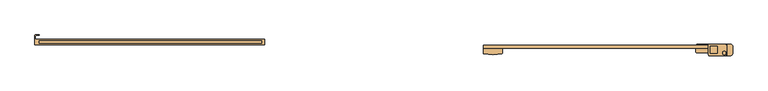
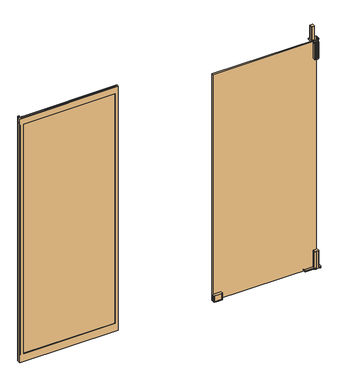
# IFC4 building model written with IfcOpenShell, lengths in millimetres: door geometry, Otomatik Kapı-Tek Kanat : Otomatik Kapı - Tek Kanat.
# Revit data of these elements (continued)
# Type "Otomatik Kapı-Tek Kanat : Otomatik Kapı - Tek Kanat" (continued)
#   Bottom Rail Note 2 [instance default] = "For the Drained continuous guide rail There must be flexible tubes on site to take out water (Slope < 1.5 %). The flexible tube connection is thread ½, and a EPDM foil or liquid synthetic material outside and a Air- and vapor-tight foil inside (on site)"
#   Bottom Rail Note [instance default] = "For drained and heated rails a cable from the header to the bottom rail in a M25 pipe is needed"
#   BIMobject category = "Sliding"
#   Assembly Code = "B2030100"
#   Analytic Construction = "<None>"
#   Standard Profile [instance default] = 5.00 cm
#   Rough Width = 313.00 cm
#   Rough Height = 220.00 cm
#   Pocket screen right = 84.07 cm
#   Pocket screen left = 84.07 cm
#   Pocket screen height [instance default] = 208.50 cm
#   Opening distance [instance default] = 0.50 cm
#   Opening Width LB = 160.00 cm
#   Opening Width Control = 160.00 cm
#   Opening Height LH = 220.00 cm
#   Moving leaf right = 80.00 cm
#   Moving leaf left = 80.00 cm
#   Moving leaf height [instance default] = 210.10 cm
#   Inset [instance default] = 0.00 cm
#   Header width = 320.00 cm
#   Header offset right CR = 0.00 cm
#   Header offset left CL = 0.00 cm
#   Header height [instance default] = 14.00 cm
#   Header Right Control = 0.00 cm
#   Header Left Control = 0.00 cm
#   Gap above header control [instance default] = 0.00 cm
#   Gap above header OH = 0.00 cm
#   Height = 220.00 cm
#   Width = 320.00 cm
#   Fixed leaf right = 80.87 cm
#   Fixed leaf left = 80.87 cm
#   Fixed leaf height [instance default] = 209.10 cm
#   CR max = 280.00 cm
#   CL max = 280.00 cm
#   Standard [instance default] = yes
#   Sideplate [instance default] = no
#   Sidecap [instance default] = no
#   Rail 4 [instance default] = no
#   Rail 3 [instance default] = no
#   Rail 2 [instance default] = no
#   Rail 1 [instance default] = no
#   Pocket screen [instance default] = yes
#   Open [instance default] = no
#   Heated [instance default] = no
#   Fixed point [instance default] = yes
#   Edition number = 1
#   Dimension Overconstraint = no
#   Connector [instance default] = no
#   Closing Profile [instance default] = no
#   Mounting Option [instance default] = element 414793
#   Mounting G = element 414798
#   Mounting F = element 414797
#   Mounting E = element 414796
#   Mounting D = element 414795
#   Mounting C = element 414794
#   Mounting B = element 414793
#   Mounting A = element 414792
#   Header Option [instance default] = element 414791
#   Header 2 = element 414791
#   Header 1 = element 414790
#   Guide 5 = element 414803
#   Guide 4 = element 414802
#   Guide 3 = element 414801
#   Guide 2 = element 414800
#   Guide 1 = element 414799
#   Frame material = Finish_Gilgen_Aluminium
#   Bottom Rail Guide [instance default] = element 414799
#   Function = (empty or 0)
#   Wall Closure = (empty or 0)
# Element 1 (IfcDoor, "Otomatik Kapı-Tek Kanat : Otomatik Kapı - Tek Kanat")
#   Materials on its faces: "Finish_Gilgen_Aluminium", "Glass", "Rubber, Natural"
# Materials
#   "Finish_Gilgen_Aluminium": class "Metal", colour RGB 120 120 120, transparency 0, Description = "Aluminium", Cost = 0
#   "Glass": class "Glass", colour RGB 0 128 192, transparency 0.9, Description = "Soda Lime Glass", Cost = 0
#   "Rubber, Natural": class "Plastic", colour RGB 120 120 120, transparency 0, Description = "Natural rubber", Cost = 0
